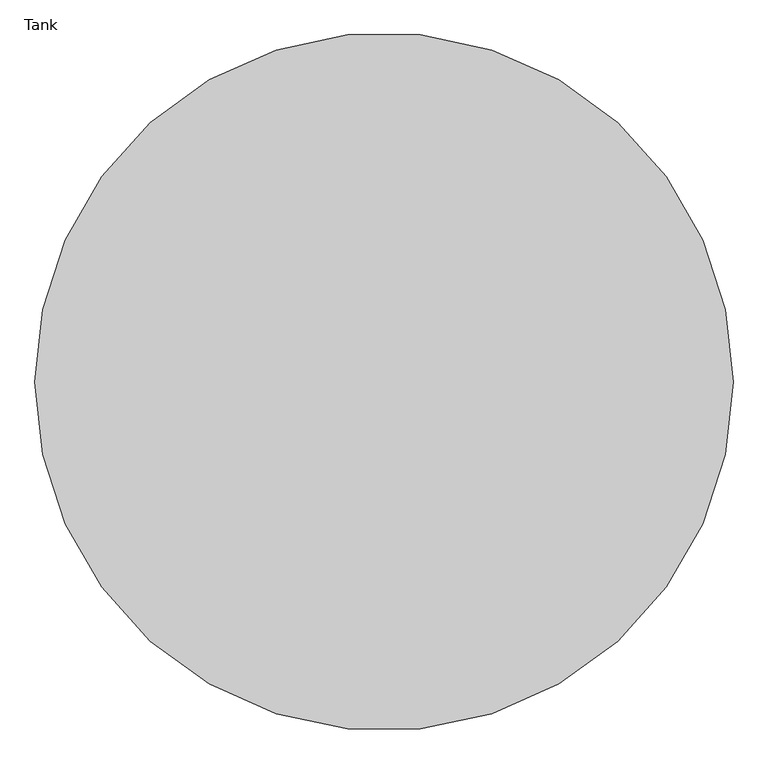
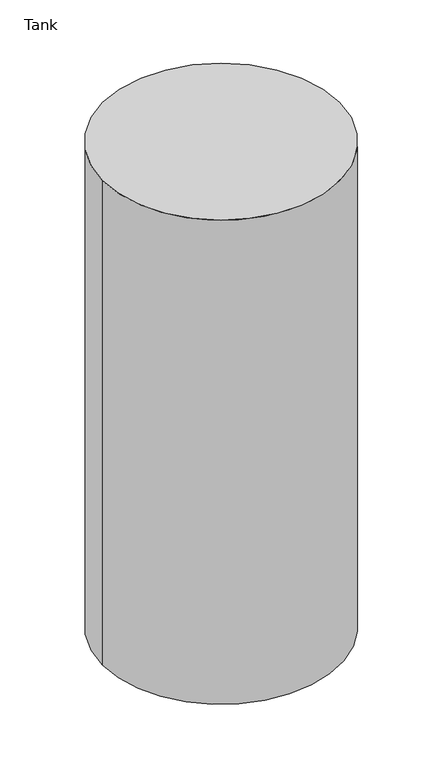
"""IFC4 building model written with IfcOpenShell, lengths in millimetres: proxy geometry, Tank : Fermenter."""

from ifc_helpers import new_model, si_unit, point, origin, origin_with_axes, origin_2d, place, context, project, spatial, circle_curve, trimmed, segment, composite_curve, outline, extrude, source, transform, mapped, element, save


def tank_f887c37f(model_context):
    return source(origin(), model_context, "Body", "SweptSolid", [
        extrude(outline(composite_curve([segment(trimmed(circle_curve(origin_2d(), 635.0), [point((-635.0, 0.0))], [point((635.0, 0.0))], False, "CARTESIAN"), True, "CONTINUOUS"), segment(trimmed(circle_curve(origin_2d(), 635.0), [point((635.0, 0.0))], [point((-635.0, 0.0))], False, "CARTESIAN"), True, "CONTINUOUS")], self_intersect=False)), origin_with_axes(), (0.0, 0.0, 1.0), 2743.2),
    ])


if __name__ == "__main__":
    model = new_model("IFC4")
    model_context = context("Model", 3, world=origin())
    ifc_project = project(units=[si_unit("LENGTHUNIT", "METRE", prefix="MILLI")], contexts=[model_context])
    site = spatial("IfcSite", under=ifc_project)
    building = spatial("IfcBuilding", under=site)
    placement = place(None, origin())
    tank_shape = tank_f887c37f(model_context)
    element("IfcBuildingElementProxy", 1, Name="Tank : Fermenter", ObjectType="Tank : Fermenter", at=placement, inside=building, context=model_context, shape_type="MappedRepresentation", body=[
        mapped(tank_shape, transform((0.0, 0.0, 0.0), x_axis=(1.0, 0.0, 0.0), y_axis=(0.0, 1.0, 0.0), z_axis=(0.0, 0.0, 1.0))),
    ])
    save(model, "model.ifc")

# Revit data of these elements
# Type "Tank : Fermenter"
#   radius = 2' - 1"
#   Height = 9' - 0"
#   Diameter = 4' - 2"
#   Material = FV (15 BBL)
# Element 1 (IfcBuildingElementProxy, "Tank : Fermenter")
#   Materials on its faces: "FV (15 BBL)"
# Materials
#   "FV (15 BBL)": class "Generic", colour RGB 181 181 181, transparency 0, Cost = 0
